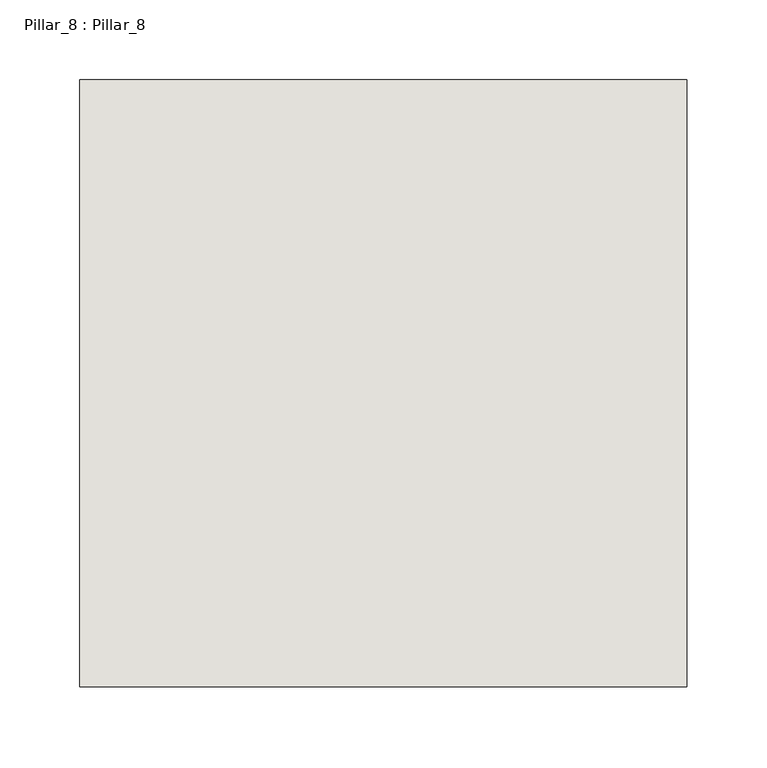
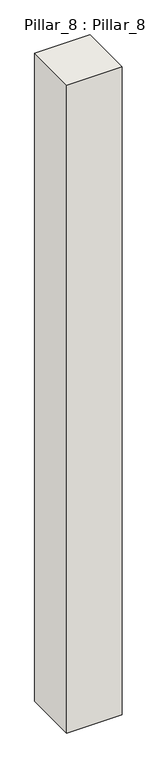
"""IFC4 building model written with IfcOpenShell, lengths in millimetres: wall geometry, Pillar_8 : Pillar_8."""

import ifcopenshell
import ifcopenshell.guid

model = None  # the IFC model being written
_history = None  # IfcOwnerHistory: only IFC2X3 demands one
_inside = {}  # id of a spatial element -> (the spatial element, [elements in it])
_under = {}  # id of a project, library or spatial element -> (it, [spatial elements below it])
_declared = {}  # id of a project -> (the project, [libraries it declares])
_typed = {}  # id of a type object -> (the type object, [elements of that type])
_made_of = {}  # id of a material, layer set ... -> (it, [elements and type objects made of it])


def new_model(schema):
    """Start an empty IFC model of exactly this schema.

    Asked for "IFC4X3", IfcOpenShell would pick the latest addendum, in which some entities
    have other attributes; the version numbers below select the first issue.
    IFC2X3 requires an IfcOwnerHistory on every rooted entity: one is made here for all.
    """
    global model, _history
    if schema == "IFC4X3":
        model = ifcopenshell.file(schema_version=(4, 3, 0, 0))
    else:
        model = ifcopenshell.file(schema=schema)
    _inside.clear()
    _under.clear()
    _declared.clear()
    _typed.clear()
    _made_of.clear()
    _history = None
    if model.schema == "IFC2X3":
        org = make("IfcOrganization", Name="unknown")
        user = make(
            "IfcPersonAndOrganization",
            ThePerson=make("IfcPerson", FamilyName="unknown"),
            TheOrganization=org,
        )
        app = make(
            "IfcApplication",
            ApplicationDeveloper=org,
            Version="unknown",
            ApplicationFullName="unknown",
            ApplicationIdentifier="unknown",
        )
        _history = make(
            "IfcOwnerHistory",
            OwningUser=user,
            OwningApplication=app,
            ChangeAction="ADDED",
            CreationDate=0,
        )
    return model


def make(cls, **values):
    """One entity of the class cls with the attributes given. An attribute that is None is left unset."""
    return model.create_entity(
        cls, **{name: value for name, value in values.items() if value is not None}
    )


def rooted(cls, **values):
    """An entity with a GlobalId (a new one), such as an element, a storey or a relation."""
    return make(cls, GlobalId=ifcopenshell.guid.new(), OwnerHistory=_history, **values)


def si_unit(unit_type, name, prefix=None):
    """IfcSIUnit, for example si_unit("LENGTHUNIT", "METRE", prefix="MILLI")."""
    return make("IfcSIUnit", UnitType=unit_type, Prefix=prefix, Name=name)


def assignment(units):
    """IfcUnitAssignment: the units of a project."""
    return None if units is None else make("IfcUnitAssignment", Units=units)


def point(xyz):
    """IfcCartesianPoint."""
    return None if xyz is None else make("IfcCartesianPoint", Coordinates=xyz)


def direction(xyz):
    """IfcDirection."""
    return None if xyz is None else make("IfcDirection", DirectionRatios=xyz)


def frame(location, z_axis=None, x_axis=None):
    """IfcAxis2Placement3D, a coordinate frame: its origin and axes. An axis left out is left unset."""
    return make(
        "IfcAxis2Placement3D",
        Location=point(location),
        Axis=direction(z_axis),
        RefDirection=direction(x_axis),
    )


def origin():
    """The frame at (0, 0, 0) with its axes left unset."""
    return frame((0.0, 0.0, 0.0))


def origin_with_axes():
    """The frame at (0, 0, 0) with the z axis (0, 0, 1) and the x axis (1, 0, 0) written out."""
    return frame((0.0, 0.0, 0.0), z_axis=(0.0, 0.0, 1.0), x_axis=(1.0, 0.0, 0.0))


def place(relative_to, where):
    """IfcLocalPlacement: puts the frame where relative to a parent placement (None: the world)."""
    return make(
        "IfcLocalPlacement", PlacementRelTo=relative_to, RelativePlacement=where
    )


def context(
    kind, dimensions, precision=None, world=None, true_north=None, identifier=None
):
    """IfcGeometricRepresentationContext, for example the 3D "Model" context."""
    return make(
        "IfcGeometricRepresentationContext",
        ContextIdentifier=identifier,
        ContextType=kind,
        CoordinateSpaceDimension=dimensions,
        Precision=precision,
        WorldCoordinateSystem=world,
        TrueNorth=true_north,
    )


def project(units=None, contexts=None):
    """IfcProject with its units and contexts."""
    return rooted(
        "IfcProject",
        Name="project",
        RepresentationContexts=contexts,
        UnitsInContext=assignment(units),
    )


def spatial(cls, under=None, at=None, **own):
    """A site, building, storey or space (cls), placed at a placement, below another one or the project."""
    s = rooted(cls, ObjectPlacement=at, **own)
    if under is not None:
        _under.setdefault(under.id(), (under, []))[1].append(s)
    return s


def polyline(points):
    """IfcPolyline through the points."""
    return make("IfcPolyline", Points=[point(p) for p in points])


def outline(outer, holes=None, kind="AREA"):
    """IfcArbitraryClosedProfileDef: a profile drawn as a closed curve; with holes, ...WithVoids."""
    if holes is None:
        return make("IfcArbitraryClosedProfileDef", ProfileType=kind, OuterCurve=outer)
    return make(
        "IfcArbitraryProfileDefWithVoids",
        ProfileType=kind,
        OuterCurve=outer,
        InnerCurves=holes,
    )


def extrude(swept, where, along, depth):
    """IfcExtrudedAreaSolid: the profile swept, set in the frame where, extruded along a direction by depth."""
    return make(
        "IfcExtrudedAreaSolid",
        SweptArea=swept,
        Position=where,
        ExtrudedDirection=direction(along),
        Depth=depth,
    )


def shape(context_of_items, identifier, shape_type, items):
    """IfcShapeRepresentation: the items that make up one representation, for example the "Body"."""
    return make(
        "IfcShapeRepresentation",
        ContextOfItems=context_of_items,
        RepresentationIdentifier=identifier,
        RepresentationType=shape_type,
        Items=items,
    )


def source(mapping_origin, context_of_items, identifier, shape_type, items):
    """IfcRepresentationMap: a shape defined once, which mapped items show again and again."""
    return make(
        "IfcRepresentationMap",
        MappingOrigin=mapping_origin,
        MappedRepresentation=shape(context_of_items, identifier, shape_type, items),
    )


def transform(
    local_origin,
    x_axis=None,
    y_axis=None,
    z_axis=None,
    scale=None,
    scale2=None,
    scale3=None,
    uniform=True,
):
    """IfcCartesianTransformationOperator3D, or its non-uniform kind. x_axis, y_axis, z_axis: its Axis1, 2, 3."""
    if uniform:
        return make(
            "IfcCartesianTransformationOperator3D",
            Axis1=direction(x_axis),
            Axis2=direction(y_axis),
            LocalOrigin=point(local_origin),
            Scale=scale,
            Axis3=direction(z_axis),
        )
    return make(
        "IfcCartesianTransformationOperator3DnonUniform",
        Axis1=direction(x_axis),
        Axis2=direction(y_axis),
        LocalOrigin=point(local_origin),
        Scale=scale,
        Axis3=direction(z_axis),
        Scale2=scale2,
        Scale3=scale3,
    )


def mapped(mapping_source, mapping_target):
    """IfcMappedItem: shows the shape of a source again, moved by a transform."""
    return make(
        "IfcMappedItem", MappingSource=mapping_source, MappingTarget=mapping_target
    )


def made_of(thing, what):
    """Note that an element or type object is made of a material, layer set ...; save() writes the relation."""
    if what is not None:
        _made_of.setdefault(what.id(), (what, []))[1].append(thing)
    return thing


def element(
    cls,
    number,
    at=None,
    inside=None,
    cuts=None,
    type_object=None,
    material=None,
    context=None,
    identifier="Body",
    shape_type=None,
    held_by="IfcProductDefinitionShape",
    body=None,
    shapes=None,
    **own,
):
    """One element of the class cls, such as IfcWall. Its Tag is "e" and its number.

    at: its placement. inside: the storey or other place that contains it. cuts: it is an
    opening in that element (IfcRelVoidsElement). A single representation is given by context,
    identifier, shape_type and body (its items); several are given by shapes. held_by: the class
    of the entity that holds the representations. save() writes the other relations.
    """
    e = rooted(cls, Tag="e%d" % number, ObjectPlacement=at, **own)
    if body is not None:
        shapes = [shape(context, identifier, shape_type, body)]
    if shapes is not None:
        e.Representation = make(held_by, Representations=shapes)
    if inside is not None:
        _inside.setdefault(inside.id(), (inside, []))[1].append(e)
    if cuts is not None:
        rooted(
            "IfcRelVoidsElement", RelatingBuildingElement=cuts, RelatedOpeningElement=e
        )
    if type_object is not None:
        _typed.setdefault(type_object.id(), (type_object, []))[1].append(e)
    return made_of(e, material)


def aggregate(whole, parts):
    """IfcRelAggregates: a whole, such as a stair, and the parts it consists of."""
    return rooted("IfcRelAggregates", RelatingObject=whole, RelatedObjects=parts)


def save(model, path):
    """Write the relations noted so far, then the file.

    IfcRelAggregates (storeys below a building ...), IfcRelContainedInSpatialStructure (elements
    in a storey), IfcRelDefinesByType, IfcRelAssociatesMaterial and IfcRelDeclares: one each for
    every whole, place, type object, material and project.
    """
    for whole, parts in _under.values():
        aggregate(whole, parts)
    for where, things in _inside.values():
        rooted(
            "IfcRelContainedInSpatialStructure",
            RelatedElements=things,
            RelatingStructure=where,
        )
    for kind, things in _typed.values():
        rooted("IfcRelDefinesByType", RelatedObjects=things, RelatingType=kind)
    for what, things in _made_of.values():
        rooted("IfcRelAssociatesMaterial", RelatedObjects=things, RelatingMaterial=what)
    for by, libraries in _declared.values():
        rooted("IfcRelDeclares", RelatingContext=by, RelatedDefinitions=libraries)
    model.write(path)


def pillar_8_pillar_8_cf5ea2e7(model_context):
    return source(origin(), model_context, "Body", "SweptSolid", [
        extrude(outline(polyline([(4060.0, 11970.0), (3680.0, 11970.0), (3680.0, 12350.0), (4060.0, 12350.0), (4060.0, 11970.0)])), origin_with_axes(), (0.0, 0.0, 1.0), 4700.0),
    ])


if __name__ == "__main__":
    model = new_model("IFC4")
    model_context = context("Model", 3, world=origin())
    ifc_project = project(units=[si_unit("LENGTHUNIT", "METRE", prefix="MILLI")], contexts=[model_context])
    site = spatial("IfcSite", under=ifc_project)
    building = spatial("IfcBuilding", under=site)
    placement = place(None, origin())
    pillar_8_pillar_8_shape = pillar_8_pillar_8_cf5ea2e7(model_context)
    element("IfcWall", 1, ObjectType="Pillar_8 : Pillar_8", at=placement, inside=building, context=model_context, shape_type="MappedRepresentation", body=[
        mapped(pillar_8_pillar_8_shape, transform((0.0, 0.0, 0.0), x_axis=(1.0, 0.0, 0.0), y_axis=(0.0, 1.0, 0.0), z_axis=(0.0, 0.0, 1.0))),
    ])
    save(model, "model.ifc")

# Revit data of these elements
# Type "Pillar_8 : Pillar_8"
#   NameOverride = "Pillar_8"
# Element 1 (IfcWall, "Pillar_8 : Pillar_8")
#   Materials on its faces: "IfcSurfaceStyle #33"
# Materials
#   "IfcSurfaceStyle #33": class "Unassigned", colour RGB 214 214 214, transparency 0
